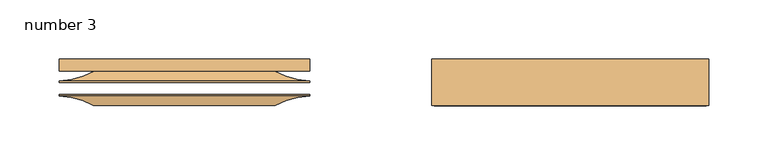
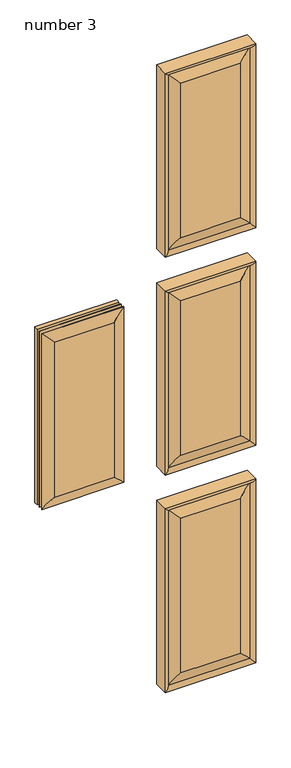
"""IFC4 building model written with IfcOpenShell, lengths in millimetres: door geometry, Door-Interior-Karona-K5660-6_Panel : number 3."""

from ifc_helpers import new_model, si_unit, frame, origin, place, context, project, spatial, polyline, ellipse_curve, source, transform, mapped, element, save
from ifc_brep_helpers import plane_surface, cylinder_surface, revolved_surface, advanced_brep


def number_3_2ed70dbe(model_context):
    return source(origin(), model_context, "Body", "AdvancedBrep", [
        advanced_brep(
        [(268.2748, 54.4576, 1893.8748), (268.2748, 54.4576, 1414.4752), (57.1627, 54.4576, 1414.4752), (57.1627, 54.4576, 1893.8748), (268.2748, 34.7218, 1893.8748), (268.2748, 36.0454899, 1893.8748), (57.1627, 36.0454899, 1893.8748), (57.1627, 34.7218, 1893.8748), (57.1627, 44.5515929, 1893.8748), (268.2748, 44.5515929, 1893.8748), (57.1627, 34.7218, 1414.4752), (57.1627, 36.0454899, 1414.4752), (268.2748, 36.0454899, 1414.4752), (268.2748, 34.7218, 1414.4752), (268.2748, 44.5515929, 1414.4752), (57.1627, 44.5515929, 1414.4752), (87.1686653, 44.5515929, 1863.8688347), (238.2688347, 44.5515929, 1863.8688347), (87.1686653, 44.5515929, 1444.4811653), (238.2688347, 44.5515929, 1444.4811653)],
        [
            (0, 1),
            (1, 2),
            (2, 3),
            (3, 0),
            (4, 5),
            (5, 6),
            (6, 7),
            (7, 4),
            (3, 8),
            (8, 9),
            (9, 0),
            (10, 11),
            (11, 12),
            (12, 13),
            (13, 10),
            (1, 14),
            (14, 15),
            (15, 2),
            (9, 14),
            (12, 5),
            (4, 13),
            (6, 11),
            (10, 7),
            (15, 8),
            (16, 6, ellipse_curve(frame((55.2243315, 100.0605261, 1895.8131685), z_axis=(-0.7071067811865475, 0.0, -0.7071067811865475), x_axis=(0.7071067811865476, 0.0, -0.7071067811865474)), 90.5724254, 64.0443762)),
            (5, 17, ellipse_curve(frame((270.2131685, 100.0605261, 1895.8131685), z_axis=(0.7071067811865475, 0.0, -0.7071067811865475), x_axis=(0.7071067811865476, 0.0, 0.7071067811865474)), 90.5724254, 64.0443762)),
            (17, 16),
            (18, 11, ellipse_curve(frame((55.2243315, 100.0605261, 1412.5368315), z_axis=(0.7071067811865475, 0.0, -0.7071067811865475), x_axis=(0.7071067811865474, 0.0, 0.7071067811865476)), 90.5724254, 64.0443762)),
            (16, 18),
            (19, 12, ellipse_curve(frame((270.2131685, 100.0605261, 1412.5368315), z_axis=(0.7071067811865475, 0.0, 0.7071067811865475), x_axis=(-0.7071067811865476, 0.0, 0.7071067811865474)), 90.5724254, 64.0443762)),
            (18, 19),
            (19, 17),
        ],
        [
            plane_surface(frame((57.1627, 54.4576, 1893.8748), z_axis=(0.0, 1.0, 0.0), x_axis=(0.0, 0.0, -1.0))),
            plane_surface(frame((57.1627, 34.7218, 1893.8748), z_axis=(0.0, 0.0, 1.0), x_axis=(-1.0, 0.0, 0.0))),
            plane_surface(frame((57.1627, 34.7218, 1414.4752), z_axis=(0.0, 0.0, -1.0), x_axis=(1.0, 0.0, 0.0))),
            plane_surface(frame((268.2748, 54.4576, 1893.8748), z_axis=(1.0, 0.0, 0.0), x_axis=(0.0, 0.0, -1.0))),
            plane_surface(frame((57.1627, 34.7218, 1893.8748), z_axis=(-1.0, 0.0, 0.0), x_axis=(0.0, 0.0, -1.0))),
            plane_surface(frame((268.2748, 34.7218, 1893.8748), z_axis=(0.0, -1.0, 0.0), x_axis=(0.0, 0.0, -1.0))),
            revolved_surface(polyline([(334.2575446888527, 100.0605261, 1831.7687923), (-8.820044688852704, 100.0605261, 1831.7687923)]), (279.4, 100.0605261, 1895.8131685), (1.0, 0.0, 0.0)),
            revolved_surface(polyline([(119.2687077, 100.0605261, 1959.8575446888528), (119.2687077, 100.0605261, 1348.4924553111473)]), (55.2243315, 100.0605261, 1905.0), (0.0, 0.0, 1.0)),
            revolved_surface(polyline([(-8.820044688852683, 100.0605261, 1476.5812077), (334.2575446888527, 100.0605261, 1476.5812077)]), (46.0375, 100.0605261, 1412.5368315), (-1.0, 0.0, 0.0)),
            revolved_surface(polyline([(206.1687923, 100.0605261, 1348.4924553111473), (206.1687923, 100.0605261, 1959.8575446888526)]), (270.2131685, 100.0605261, 1403.35), (0.0, 0.0, -1.0)),
            plane_surface(frame((279.4, 44.5515929, 1403.35), z_axis=(0.0, -1.0, 0.0), x_axis=(0.0, 0.0, 1.0))),
        ],
        [
            (0, [[1, 2, 3, 4]]),
            (1, [[5, 6, 7, 8]]),
            (1, [[9, 10, 11, -4]]),
            (2, [[12, 13, 14, 15]]),
            (2, [[16, 17, 18, -2]]),
            (3, [[-11, 19, -16, -1]]),
            (3, [[-14, 20, -5, 21]]),
            (4, [[-7, 22, -12, 23]]),
            (4, [[-18, 24, -9, -3]]),
            (5, [[-23, -15, -21, -8]]),
            (6, [[25, -6, 26, 27]]),
            (7, [[28, -22, -25, 29]]),
            (8, [[30, -13, -28, 31]]),
            (9, [[-26, -20, -30, 32]]),
            (10, [[-24, -17, -19, -10], [-32, -31, -29, -27]]),
        ],
    ),
        advanced_brep(
        [(268.2748, 24.6126, 1893.8748), (268.2748, 24.6126, 1414.4752), (57.1627, 24.6126, 1414.4752), (57.1627, 24.6126, 1893.8748), (239.4448579, 15.4432, 1443.3051421), (239.4448579, 15.4432, 1865.0448579), (85.9926421, 15.4432, 1865.0448579), (85.9926421, 15.4432, 1443.3051421), (57.1627, 23.2889101, 1893.8748), (268.2748, 23.2889101, 1893.8748), (268.2748, 23.2889101, 1414.4752), (57.1627, 23.2889101, 1414.4752)],
        [
            (0, 1),
            (1, 2),
            (2, 3),
            (3, 0),
            (4, 5),
            (5, 6),
            (6, 7),
            (7, 4),
            (3, 8),
            (8, 9),
            (9, 0),
            (1, 10),
            (10, 11),
            (11, 2),
            (7, 11, ellipse_curve(frame((55.2243315, -40.7261261, 1412.5368315), z_axis=(-0.7071067811865475, 0.0, 0.7071067811865475), x_axis=(-0.7071067811865476, 0.0, -0.7071067811865474)), 90.5724254, 64.0443762)),
            (10, 4, ellipse_curve(frame((270.2131685, -40.7261261, 1412.5368315), z_axis=(0.7071067811865475, 0.0, 0.7071067811865475), x_axis=(-0.7071067811865476, 0.0, 0.7071067811865474)), 90.5724254, 64.0443762)),
            (10, 9),
            (9, 5, ellipse_curve(frame((270.2131685, -40.7261261, 1895.8131685), z_axis=(-0.7071067811865475, 0.0, 0.7071067811865475), x_axis=(-0.7071067811865474, 0.0, -0.7071067811865476)), 90.5724254, 64.0443762)),
            (8, 6, ellipse_curve(frame((55.2243315, -40.7261261, 1895.8131685), z_axis=(-0.7071067811865475, 0.0, -0.7071067811865475), x_axis=(0.7071067811865476, 0.0, -0.7071067811865474)), 90.5724254, 64.0443762)),
            (8, 11),
        ],
        [
            plane_surface(frame((57.1627, 24.6126, 1893.8748), z_axis=(0.0, 1.0, 0.0), x_axis=(0.0, 0.0, -1.0))),
            plane_surface(frame((268.2748, 15.4432, 1893.8748), z_axis=(0.0, -1.0, 0.0), x_axis=(0.0, 0.0, -1.0))),
            plane_surface(frame((57.1627, 34.7218, 1893.8748), z_axis=(0.0, 0.0, 1.0), x_axis=(-1.0, 0.0, 0.0))),
            plane_surface(frame((57.1627, 34.7218, 1414.4752), z_axis=(0.0, 0.0, -1.0), x_axis=(1.0, 0.0, 0.0))),
            revolved_surface(polyline([(-8.820044688852711, -40.7261261, 1476.5812077), (334.2575446888527, -40.7261261, 1476.5812077)]), (46.0375, -40.7261261, 1412.5368315), (-1.0, 0.0, 0.0)),
            revolved_surface(polyline([(206.1687923, -40.7261261, 1348.4924553111473), (206.1687923, -40.7261261, 1959.8575446888528)]), (270.2131685, -40.7261261, 1403.35), (0.0, 0.0, -1.0)),
            revolved_surface(polyline([(334.2575446888527, -40.7261261, 1831.7687923), (-8.820044688852704, -40.7261261, 1831.7687923)]), (279.4, -40.7261261, 1895.8131685), (1.0, 0.0, 0.0)),
            revolved_surface(polyline([(119.2687077, -40.7261261, 1959.8575446888528), (119.2687077, -40.7261261, 1348.4924553111473)]), (55.2243315, -40.7261261, 1905.0), (0.0, 0.0, 1.0)),
            plane_surface(frame((268.2748, 24.6126, 1893.8748), z_axis=(1.0, 0.0, 0.0), x_axis=(0.0, 0.0, -1.0))),
            plane_surface(frame((57.1627, 15.4432, 1893.8748), z_axis=(-1.0, 0.0, 0.0), x_axis=(0.0, 0.0, -1.0))),
        ],
        [
            (0, [[1, 2, 3, 4]]),
            (1, [[5, 6, 7, 8]]),
            (2, [[9, 10, 11, -4]]),
            (3, [[12, 13, 14, -2]]),
            (4, [[-8, 15, -13, 16]]),
            (5, [[17, 18, -5, -16]]),
            (6, [[-10, 19, -6, -18]]),
            (7, [[20, -15, -7, -19]]),
            (8, [[-11, -17, -12, -1]]),
            (9, [[-14, -20, -9, -3]]),
        ],
    ),
        advanced_brep(
        [(279.4, 15.2908, 1905.0), (46.0375, 15.2908, 1905.0), (57.3628137, 24.6126, 1893.6746863), (268.0746863, 24.6126, 1893.6746863), (57.1627, 46.3324899, 1893.8748), (57.1627, 46.3324899, 1414.4752), (48.2727, 54.4576, 1405.5852), (48.2727, 54.4576, 1902.7648), (268.2748, 46.3324899, 1414.4752), (268.2748, 46.3324899, 1893.8748), (277.1648, 54.4576, 1902.7648), (277.1648, 54.4576, 1405.5852), (46.0375, 54.4576, 1403.35), (279.4, 54.4576, 1403.35), (279.4, 15.2908, 1403.35), (46.0375, 15.2908, 1403.35), (57.1627, 34.7218, 1414.4752), (268.2748, 34.7218, 1414.4752), (47.3075, 24.6126, 1903.73), (47.3075, 24.6126, 1404.62), (47.3075, 34.7218, 1404.62), (47.3075, 34.7218, 1903.73), (278.13, 24.6126, 1404.62), (278.13, 24.6126, 1903.73), (57.3628137, 24.6126, 1414.6753137), (268.0746863, 24.6126, 1414.6753137), (278.13, 34.7218, 1404.62), (279.4, 54.4576, 1905.0), (268.2748, 34.7218, 1893.8748), (278.13, 34.7218, 1903.73), (46.0375, 54.4576, 1905.0), (57.1627, 34.7218, 1893.8748)],
        [
            (0, 1),
            (1, 2, ellipse_curve(frame((47.0685124, 25.5788135, 1903.9689876), z_axis=(0.7071067811865475, 0.0, 0.7071067811865475), x_axis=(0.7071067811865476, 0.0, -0.7071067811865474)), 14.6223259, 10.3395458)),
            (2, 3),
            (3, 0, ellipse_curve(frame((278.3689876, 25.5788135, 1903.9689876), z_axis=(-0.7071067811865475, 0.0, 0.7071067811865475), x_axis=(0.7071067811865476, 0.0, 0.7071067811865474)), 14.6223259, 10.3395458)),
            (4, 5),
            (5, 6, ellipse_curve(frame((48.2727, 45.531597, 1405.5852), z_axis=(-0.7071067811865475, 0.0, 0.7071067811865475), x_axis=(0.7071067811865474, 0.0, 0.7071067811865476)), 12.6232745, 8.926003)),
            (6, 7),
            (7, 4, ellipse_curve(frame((48.2727, 45.531597, 1902.7648), z_axis=(-0.7071067811865475, 0.0, -0.7071067811865475), x_axis=(-0.7071067811865474, 0.0, 0.7071067811865476)), 12.6232745, 8.926003)),
            (8, 9),
            (9, 10, ellipse_curve(frame((277.1648, 45.531597, 1902.7648), z_axis=(0.7071067811865475, 0.0, -0.7071067811865475), x_axis=(-0.7071067811865474, 0.0, -0.7071067811865476)), 12.6232745, 8.926003)),
            (10, 11),
            (11, 8, ellipse_curve(frame((277.1648, 45.531597, 1405.5852), z_axis=(0.7071067811865475, 0.0, 0.7071067811865475), x_axis=(0.7071067811865474, 0.0, -0.7071067811865476)), 12.6232745, 8.926003)),
            (12, 13),
            (13, 14),
            (14, 15),
            (15, 12),
            (16, 17),
            (17, 8),
            (8, 5),
            (5, 16),
            (18, 19),
            (19, 20),
            (20, 21),
            (21, 18),
            (22, 19),
            (18, 23),
            (23, 22),
            (24, 25),
            (25, 3),
            (2, 24),
            (22, 26),
            (26, 20),
            (13, 27),
            (27, 0),
            (0, 14),
            (17, 28),
            (28, 9),
            (23, 29),
            (29, 26),
            (27, 30),
            (30, 1),
            (28, 31),
            (31, 4),
            (4, 9),
            (21, 29),
            (30, 12),
            (15, 1),
            (31, 16),
            (6, 11),
            (10, 7),
            (14, 25, ellipse_curve(frame((278.3689876, 25.5788135, 1404.3810124), z_axis=(-0.7071067811865475, 0.0, -0.7071067811865475), x_axis=(-0.7071067811865476, 0.0, 0.7071067811865474)), 14.6223259, 10.3395458)),
            (24, 15, ellipse_curve(frame((47.0685124, 25.5788135, 1404.3810124), z_axis=(0.7071067811865475, 0.0, -0.7071067811865475), x_axis=(-0.7071067811865476, 0.0, -0.7071067811865474)), 14.6223259, 10.3395458)),
        ],
        [
            cylinder_surface(frame((279.4, 25.5788135, 1903.9689876), z_axis=(1.0, 0.0, 0.0), x_axis=(0.0, -1.0, 0.0)), 10.3395458),
            cylinder_surface(frame((48.2727, 45.531597, 1905.0), z_axis=(0.0, 0.0, 1.0), x_axis=(0.0, -1.0, 0.0)), 8.926003),
            cylinder_surface(frame((277.1648, 45.531597, 1403.35), z_axis=(0.0, 0.0, -1.0), x_axis=(0.0, -1.0, 0.0)), 8.926003),
            plane_surface(frame((46.0375, 15.2908, 1403.35), z_axis=(0.0, 0.0, -1.0), x_axis=(1.0, 0.0, 0.0))),
            plane_surface(frame((57.1627, 46.3324899, 1414.4752), z_axis=(0.0, 0.0, 1.0), x_axis=(1.0, 0.0, 0.0))),
            plane_surface(frame((47.3075, 34.7218, 1903.73), z_axis=(1.0, 0.0, 0.0), x_axis=(0.0, 0.0, -1.0))),
            plane_surface(frame((47.3075, 24.6126, 1903.73), z_axis=(0.0, 1.0, 0.0), x_axis=(0.0, 0.0, -1.0))),
            plane_surface(frame((47.3075, 34.7218, 1404.62), z_axis=(0.0, 0.0, 1.0), x_axis=(1.0, 0.0, 0.0))),
            plane_surface(frame((279.4, 15.2908, 1403.35), z_axis=(1.0, 0.0, 0.0), x_axis=(0.0, 0.0, 1.0))),
            plane_surface(frame((268.2748, 46.3324899, 1414.4752), z_axis=(-1.0, 0.0, 0.0), x_axis=(0.0, 0.0, 1.0))),
            plane_surface(frame((278.13, 34.7218, 1404.62), z_axis=(-1.0, 0.0, 0.0), x_axis=(0.0, 0.0, 1.0))),
            plane_surface(frame((279.4, 15.2908, 1905.0), z_axis=(0.0, 0.0, 1.0), x_axis=(-1.0, 0.0, 0.0))),
            plane_surface(frame((268.2748, 46.3324899, 1893.8748), z_axis=(0.0, 0.0, -1.0), x_axis=(-1.0, 0.0, 0.0))),
            plane_surface(frame((278.13, 34.7218, 1903.73), z_axis=(0.0, 0.0, -1.0), x_axis=(-1.0, 0.0, 0.0))),
            plane_surface(frame((46.0375, 15.2908, 1905.0), z_axis=(-1.0, 0.0, 0.0), x_axis=(0.0, 0.0, -1.0))),
            plane_surface(frame((57.1627, 46.3324899, 1893.8748), z_axis=(1.0, 0.0, 0.0), x_axis=(0.0, 0.0, -1.0))),
            plane_surface(frame((57.1627, 34.7218, 1893.8748), z_axis=(0.0, -1.0, 0.0), x_axis=(0.0, 0.0, -1.0))),
            plane_surface(frame((46.0375, 54.4576, 1905.0), z_axis=(0.0, 1.0, 0.0), x_axis=(0.0, 0.0, -1.0))),
            cylinder_surface(frame((46.0375, 45.531597, 1405.5852), z_axis=(-1.0, 0.0, 0.0), x_axis=(0.0, -1.0, 0.0)), 8.926003),
            cylinder_surface(frame((46.0375, 25.5788135, 1404.3810124), z_axis=(-1.0, 0.0, 0.0), x_axis=(0.0, -1.0, 0.0)), 10.3395458),
            cylinder_surface(frame((278.3689876, 25.5788135, 1403.35), z_axis=(0.0, 0.0, -1.0), x_axis=(0.0, -1.0, 0.0)), 10.3395458),
            cylinder_surface(frame((279.4, 45.531597, 1902.7648), z_axis=(1.0, 0.0, 0.0), x_axis=(0.0, -1.0, 0.0)), 8.926003),
            cylinder_surface(frame((47.0685124, 25.5788135, 1905.0), z_axis=(0.0, 0.0, 1.0), x_axis=(0.0, -1.0, 0.0)), 10.3395458),
        ],
        [
            (0, [[1, 2, 3, 4]]),
            (1, [[5, 6, 7, 8]]),
            (2, [[9, 10, 11, 12]]),
            (3, [[13, 14, 15, 16]]),
            (4, [[17, 18, 19, 20]]),
            (5, [[21, 22, 23, 24]]),
            (6, [[25, -21, 26, 27], [28, 29, -3, 30]]),
            (7, [[-25, 31, 32, -22]]),
            (8, [[33, 34, 35, -14]]),
            (9, [[36, 37, -9, -18]]),
            (10, [[-27, 38, 39, -31]]),
            (11, [[40, 41, -1, -34]]),
            (12, [[42, 43, 44, -37]]),
            (13, [[-26, -24, 45, -38]]),
            (14, [[46, -16, 47, -41]]),
            (15, [[48, -20, -5, -43]]),
            (16, [[-32, -39, -45, -23], [-17, -48, -42, -36]]),
            (17, [[-13, -46, -40, -33], [49, -11, 50, -7]]),
            (18, [[-19, -12, -49, -6]]),
            (19, [[-15, 51, -28, 52]]),
            (20, [[-35, -4, -29, -51]]),
            (21, [[-44, -8, -50, -10]]),
            (22, [[-47, -52, -30, -2]]),
        ],
    ),
        advanced_brep(
        [(268.2748, 54.4576, 1300.1498), (268.2748, 54.4576, 820.7502), (57.1627, 54.4576, 820.7502), (57.1627, 54.4576, 1300.1498), (268.2748, 34.7218, 1300.1498), (268.2748, 36.0454899, 1300.1498), (57.1627, 36.0454899, 1300.1498), (57.1627, 34.7218, 1300.1498), (57.1627, 44.5515929, 1300.1498), (268.2748, 44.5515929, 1300.1498), (57.1627, 34.7218, 820.7502), (57.1627, 36.0454899, 820.7502), (268.2748, 36.0454899, 820.7502), (268.2748, 34.7218, 820.7502), (268.2748, 44.5515929, 820.7502), (57.1627, 44.5515929, 820.7502), (87.1686653, 44.5515929, 1270.1438347), (238.2688347, 44.5515929, 1270.1438347), (87.1686653, 44.5515929, 850.7561653), (238.2688347, 44.5515929, 850.7561653)],
        [
            (0, 1),
            (1, 2),
            (2, 3),
            (3, 0),
            (4, 5),
            (5, 6),
            (6, 7),
            (7, 4),
            (3, 8),
            (8, 9),
            (9, 0),
            (10, 11),
            (11, 12),
            (12, 13),
            (13, 10),
            (1, 14),
            (14, 15),
            (15, 2),
            (9, 14),
            (12, 5),
            (4, 13),
            (6, 11),
            (10, 7),
            (15, 8),
            (16, 6, ellipse_curve(frame((55.2243315, 100.0605261, 1302.0881685), z_axis=(-0.7071067811865475, 0.0, -0.7071067811865475), x_axis=(0.7071067811865476, 0.0, -0.7071067811865474)), 90.5724254, 64.0443762)),
            (5, 17, ellipse_curve(frame((270.2131685, 100.0605261, 1302.0881685), z_axis=(0.7071067811865475, 0.0, -0.7071067811865475), x_axis=(0.7071067811865476, 0.0, 0.7071067811865474)), 90.5724254, 64.0443762)),
            (17, 16),
            (18, 11, ellipse_curve(frame((55.2243315, 100.0605261, 818.8118315), z_axis=(0.7071067811865475, 0.0, -0.7071067811865475), x_axis=(0.7071067811865474, 0.0, 0.7071067811865476)), 90.5724254, 64.0443762)),
            (16, 18),
            (19, 12, ellipse_curve(frame((270.2131685, 100.0605261, 818.8118315), z_axis=(0.7071067811865475, 0.0, 0.7071067811865475), x_axis=(-0.7071067811865476, 0.0, 0.7071067811865474)), 90.5724254, 64.0443762)),
            (18, 19),
            (19, 17),
        ],
        [
            plane_surface(frame((57.1627, 54.4576, 1300.1498), z_axis=(0.0, 1.0, 0.0), x_axis=(0.0, 0.0, -1.0))),
            plane_surface(frame((57.1627, 34.7218, 1300.1498), z_axis=(0.0, 0.0, 1.0), x_axis=(-1.0, 0.0, 0.0))),
            plane_surface(frame((57.1627, 34.7218, 820.7502), z_axis=(0.0, 0.0, -1.0), x_axis=(1.0, 0.0, 0.0))),
            plane_surface(frame((268.2748, 54.4576, 1300.1498), z_axis=(1.0, 0.0, 0.0), x_axis=(0.0, 0.0, -1.0))),
            plane_surface(frame((57.1627, 34.7218, 1300.1498), z_axis=(-1.0, 0.0, 0.0), x_axis=(0.0, 0.0, -1.0))),
            plane_surface(frame((268.2748, 34.7218, 1300.1498), z_axis=(0.0, -1.0, 0.0), x_axis=(0.0, 0.0, -1.0))),
            revolved_surface(polyline([(334.2575446888527, 100.0605261, 1238.0437923), (-8.820044688852704, 100.0605261, 1238.0437923)]), (279.4, 100.0605261, 1302.0881685), (1.0, 0.0, 0.0)),
            revolved_surface(polyline([(119.2687077, 100.0605261, 1366.1325446888527), (119.2687077, 100.0605261, 754.7674553111474)]), (55.2243315, 100.0605261, 1311.275), (0.0, 0.0, 1.0)),
            revolved_surface(polyline([(-8.820044688852683, 100.0605261, 882.8562077), (334.2575446888527, 100.0605261, 882.8562077)]), (46.0375, 100.0605261, 818.8118315), (-1.0, 0.0, 0.0)),
            revolved_surface(polyline([(206.1687923, 100.0605261, 754.7674553111474), (206.1687923, 100.0605261, 1366.1325446888527)]), (270.2131685, 100.0605261, 809.625), (0.0, 0.0, -1.0)),
            plane_surface(frame((279.4, 44.5515929, 809.625), z_axis=(0.0, -1.0, 0.0), x_axis=(0.0, 0.0, 1.0))),
        ],
        [
            (0, [[1, 2, 3, 4]]),
            (1, [[5, 6, 7, 8]]),
            (1, [[9, 10, 11, -4]]),
            (2, [[12, 13, 14, 15]]),
            (2, [[16, 17, 18, -2]]),
            (3, [[-11, 19, -16, -1]]),
            (3, [[-14, 20, -5, 21]]),
            (4, [[-7, 22, -12, 23]]),
            (4, [[-18, 24, -9, -3]]),
            (5, [[-23, -15, -21, -8]]),
            (6, [[25, -6, 26, 27]]),
            (7, [[28, -22, -25, 29]]),
            (8, [[30, -13, -28, 31]]),
            (9, [[-26, -20, -30, 32]]),
            (10, [[-24, -17, -19, -10], [-32, -31, -29, -27]]),
        ],
    ),
        advanced_brep(
        [(268.2748, 24.6126, 1300.1498), (268.2748, 24.6126, 820.7502), (57.1627, 24.6126, 820.7502), (57.1627, 24.6126, 1300.1498), (239.4448579, 15.4432, 849.5801421), (239.4448579, 15.4432, 1271.3198579), (85.9926421, 15.4432, 1271.3198579), (85.9926421, 15.4432, 849.5801421), (57.1627, 23.2889101, 1300.1498), (268.2748, 23.2889101, 1300.1498), (268.2748, 23.2889101, 820.7502), (57.1627, 23.2889101, 820.7502)],
        [
            (0, 1),
            (1, 2),
            (2, 3),
            (3, 0),
            (4, 5),
            (5, 6),
            (6, 7),
            (7, 4),
            (3, 8),
            (8, 9),
            (9, 0),
            (1, 10),
            (10, 11),
            (11, 2),
            (7, 11, ellipse_curve(frame((55.2243315, -40.7261261, 818.8118315), z_axis=(-0.7071067811865475, 0.0, 0.7071067811865475), x_axis=(-0.7071067811865476, 0.0, -0.7071067811865474)), 90.5724254, 64.0443762)),
            (10, 4, ellipse_curve(frame((270.2131685, -40.7261261, 818.8118315), z_axis=(0.7071067811865475, 0.0, 0.7071067811865475), x_axis=(-0.7071067811865476, 0.0, 0.7071067811865474)), 90.5724254, 64.0443762)),
            (10, 9),
            (9, 5, ellipse_curve(frame((270.2131685, -40.7261261, 1302.0881685), z_axis=(-0.7071067811865475, 0.0, 0.7071067811865475), x_axis=(-0.7071067811865474, 0.0, -0.7071067811865476)), 90.5724254, 64.0443762)),
            (8, 6, ellipse_curve(frame((55.2243315, -40.7261261, 1302.0881685), z_axis=(-0.7071067811865475, 0.0, -0.7071067811865475), x_axis=(0.7071067811865476, 0.0, -0.7071067811865474)), 90.5724254, 64.0443762)),
            (8, 11),
        ],
        [
            plane_surface(frame((57.1627, 24.6126, 1300.1498), z_axis=(0.0, 1.0, 0.0), x_axis=(0.0, 0.0, -1.0))),
            plane_surface(frame((268.2748, 15.4432, 1300.1498), z_axis=(0.0, -1.0, 0.0), x_axis=(0.0, 0.0, -1.0))),
            plane_surface(frame((57.1627, 34.7218, 1300.1498), z_axis=(0.0, 0.0, 1.0), x_axis=(-1.0, 0.0, 0.0))),
            plane_surface(frame((57.1627, 34.7218, 820.7502), z_axis=(0.0, 0.0, -1.0), x_axis=(1.0, 0.0, 0.0))),
            revolved_surface(polyline([(-8.820044688852711, -40.7261261, 882.8562077), (334.2575446888527, -40.7261261, 882.8562077)]), (46.0375, -40.7261261, 818.8118315), (-1.0, 0.0, 0.0)),
            revolved_surface(polyline([(206.1687923, -40.7261261, 754.7674553111474), (206.1687923, -40.7261261, 1366.1325446888527)]), (270.2131685, -40.7261261, 809.625), (0.0, 0.0, -1.0)),
            revolved_surface(polyline([(334.2575446888527, -40.7261261, 1238.0437923), (-8.820044688852704, -40.7261261, 1238.0437923)]), (279.4, -40.7261261, 1302.0881685), (1.0, 0.0, 0.0)),
            revolved_surface(polyline([(119.2687077, -40.7261261, 1366.1325446888527), (119.2687077, -40.7261261, 754.7674553111474)]), (55.2243315, -40.7261261, 1311.275), (0.0, 0.0, 1.0)),
            plane_surface(frame((268.2748, 24.6126, 1300.1498), z_axis=(1.0, 0.0, 0.0), x_axis=(0.0, 0.0, -1.0))),
            plane_surface(frame((57.1627, 15.4432, 1300.1498), z_axis=(-1.0, 0.0, 0.0), x_axis=(0.0, 0.0, -1.0))),
        ],
        [
            (0, [[1, 2, 3, 4]]),
            (1, [[5, 6, 7, 8]]),
            (2, [[9, 10, 11, -4]]),
            (3, [[12, 13, 14, -2]]),
            (4, [[-8, 15, -13, 16]]),
            (5, [[17, 18, -5, -16]]),
            (6, [[-10, 19, -6, -18]]),
            (7, [[20, -15, -7, -19]]),
            (8, [[-11, -17, -12, -1]]),
            (9, [[-14, -20, -9, -3]]),
        ],
    ),
        advanced_brep(
        [(279.4, 15.2908, 1311.275), (46.0375, 15.2908, 1311.275), (57.3628137, 24.6126, 1299.9496863), (268.0746863, 24.6126, 1299.9496863), (57.1627, 46.3324899, 1300.1498), (57.1627, 46.3324899, 820.7502), (48.2727, 54.4576, 811.8602), (48.2727, 54.4576, 1309.0398), (268.2748, 46.3324899, 820.7502), (268.2748, 46.3324899, 1300.1498), (277.1648, 54.4576, 1309.0398), (277.1648, 54.4576, 811.8602), (46.0375, 54.4576, 809.625), (279.4, 54.4576, 809.625), (279.4, 15.2908, 809.625), (46.0375, 15.2908, 809.625), (57.1627, 34.7218, 820.7502), (268.2748, 34.7218, 820.7502), (47.3075, 24.6126, 1310.005), (47.3075, 24.6126, 810.895), (47.3075, 34.7218, 810.895), (47.3075, 34.7218, 1310.005), (278.13, 24.6126, 810.895), (278.13, 24.6126, 1310.005), (57.3628137, 24.6126, 820.9503137), (268.0746863, 24.6126, 820.9503137), (278.13, 34.7218, 810.895), (279.4, 54.4576, 1311.275), (268.2748, 34.7218, 1300.1498), (278.13, 34.7218, 1310.005), (46.0375, 54.4576, 1311.275), (57.1627, 34.7218, 1300.1498)],
        [
            (0, 1),
            (1, 2, ellipse_curve(frame((47.0685124, 25.5788135, 1310.2439876), z_axis=(0.7071067811865475, 0.0, 0.7071067811865475), x_axis=(0.7071067811865476, 0.0, -0.7071067811865474)), 14.6223259, 10.3395458)),
            (2, 3),
            (3, 0, ellipse_curve(frame((278.3689876, 25.5788135, 1310.2439876), z_axis=(-0.7071067811865475, 0.0, 0.7071067811865475), x_axis=(0.7071067811865476, 0.0, 0.7071067811865474)), 14.6223259, 10.3395458)),
            (4, 5),
            (5, 6, ellipse_curve(frame((48.2727, 45.531597, 811.8602), z_axis=(-0.7071067811865475, 0.0, 0.7071067811865475), x_axis=(0.7071067811865474, 0.0, 0.7071067811865476)), 12.6232745, 8.926003)),
            (6, 7),
            (7, 4, ellipse_curve(frame((48.2727, 45.531597, 1309.0398), z_axis=(-0.7071067811865475, 0.0, -0.7071067811865475), x_axis=(-0.7071067811865474, 0.0, 0.7071067811865476)), 12.6232745, 8.926003)),
            (8, 9),
            (9, 10, ellipse_curve(frame((277.1648, 45.531597, 1309.0398), z_axis=(0.7071067811865475, 0.0, -0.7071067811865475), x_axis=(-0.7071067811865474, 0.0, -0.7071067811865476)), 12.6232745, 8.926003)),
            (10, 11),
            (11, 8, ellipse_curve(frame((277.1648, 45.531597, 811.8602), z_axis=(0.7071067811865475, 0.0, 0.7071067811865475), x_axis=(0.7071067811865474, 0.0, -0.7071067811865476)), 12.6232745, 8.926003)),
            (12, 13),
            (13, 14),
            (14, 15),
            (15, 12),
            (16, 17),
            (17, 8),
            (8, 5),
            (5, 16),
            (18, 19),
            (19, 20),
            (20, 21),
            (21, 18),
            (22, 19),
            (18, 23),
            (23, 22),
            (24, 25),
            (25, 3),
            (2, 24),
            (14, 25, ellipse_curve(frame((278.3689876, 25.5788135, 810.6560124), z_axis=(-0.7071067811865475, 0.0, -0.7071067811865475), x_axis=(-0.7071067811865476, 0.0, 0.7071067811865474)), 14.6223259, 10.3395458)),
            (24, 15, ellipse_curve(frame((47.0685124, 25.5788135, 810.6560124), z_axis=(0.7071067811865475, 0.0, -0.7071067811865475), x_axis=(-0.7071067811865476, 0.0, -0.7071067811865474)), 14.6223259, 10.3395458)),
            (22, 26),
            (26, 20),
            (13, 27),
            (27, 0),
            (0, 14),
            (17, 28),
            (28, 9),
            (23, 29),
            (29, 26),
            (27, 30),
            (30, 1),
            (28, 31),
            (31, 4),
            (4, 9),
            (21, 29),
            (30, 12),
            (15, 1),
            (31, 16),
            (6, 11),
            (10, 7),
        ],
        [
            cylinder_surface(frame((279.4, 25.5788135, 1310.2439876), z_axis=(1.0, 0.0, 0.0), x_axis=(0.0, -1.0, 0.0)), 10.3395458),
            cylinder_surface(frame((48.2727, 45.531597, 1311.275), z_axis=(0.0, 0.0, 1.0), x_axis=(0.0, -1.0, 0.0)), 8.926003),
            cylinder_surface(frame((277.1648, 45.531597, 809.625), z_axis=(0.0, 0.0, -1.0), x_axis=(0.0, -1.0, 0.0)), 8.926003),
            plane_surface(frame((46.0375, 15.2908, 809.625), z_axis=(0.0, 0.0, -1.0), x_axis=(1.0, 0.0, 0.0))),
            plane_surface(frame((57.1627, 46.3324899, 820.7502), z_axis=(0.0, 0.0, 1.0), x_axis=(1.0, 0.0, 0.0))),
            plane_surface(frame((47.3075, 34.7218, 1310.005), z_axis=(1.0, 0.0, 0.0), x_axis=(0.0, 0.0, -1.0))),
            plane_surface(frame((47.3075, 24.6126, 1310.005), z_axis=(0.0, 1.0, 0.0), x_axis=(0.0, 0.0, -1.0))),
            cylinder_surface(frame((46.0375, 25.5788135, 810.6560124), z_axis=(-1.0, 0.0, 0.0), x_axis=(0.0, -1.0, 0.0)), 10.3395458),
            plane_surface(frame((47.3075, 34.7218, 810.895), z_axis=(0.0, 0.0, 1.0), x_axis=(1.0, 0.0, 0.0))),
            plane_surface(frame((279.4, 15.2908, 809.625), z_axis=(1.0, 0.0, 0.0), x_axis=(0.0, 0.0, 1.0))),
            plane_surface(frame((268.2748, 46.3324899, 820.7502), z_axis=(-1.0, 0.0, 0.0), x_axis=(0.0, 0.0, 1.0))),
            plane_surface(frame((278.13, 34.7218, 810.895), z_axis=(-1.0, 0.0, 0.0), x_axis=(0.0, 0.0, 1.0))),
            plane_surface(frame((279.4, 15.2908, 1311.275), z_axis=(0.0, 0.0, 1.0), x_axis=(-1.0, 0.0, 0.0))),
            plane_surface(frame((268.2748, 46.3324899, 1300.1498), z_axis=(0.0, 0.0, -1.0), x_axis=(-1.0, 0.0, 0.0))),
            plane_surface(frame((278.13, 34.7218, 1310.005), z_axis=(0.0, 0.0, -1.0), x_axis=(-1.0, 0.0, 0.0))),
            plane_surface(frame((46.0375, 15.2908, 1311.275), z_axis=(-1.0, 0.0, 0.0), x_axis=(0.0, 0.0, -1.0))),
            plane_surface(frame((57.1627, 46.3324899, 1300.1498), z_axis=(1.0, 0.0, 0.0), x_axis=(0.0, 0.0, -1.0))),
            plane_surface(frame((57.1627, 34.7218, 1300.1498), z_axis=(0.0, -1.0, 0.0), x_axis=(0.0, 0.0, -1.0))),
            plane_surface(frame((46.0375, 54.4576, 1311.275), z_axis=(0.0, 1.0, 0.0), x_axis=(0.0, 0.0, -1.0))),
            cylinder_surface(frame((46.0375, 45.531597, 811.8602), z_axis=(-1.0, 0.0, 0.0), x_axis=(0.0, -1.0, 0.0)), 8.926003),
            cylinder_surface(frame((278.3689876, 25.5788135, 809.625), z_axis=(0.0, 0.0, -1.0), x_axis=(0.0, -1.0, 0.0)), 10.3395458),
            cylinder_surface(frame((279.4, 45.531597, 1309.0398), z_axis=(1.0, 0.0, 0.0), x_axis=(0.0, -1.0, 0.0)), 8.926003),
            cylinder_surface(frame((47.0685124, 25.5788135, 1311.275), z_axis=(0.0, 0.0, 1.0), x_axis=(0.0, -1.0, 0.0)), 10.3395458),
        ],
        [
            (0, [[1, 2, 3, 4]]),
            (1, [[5, 6, 7, 8]]),
            (2, [[9, 10, 11, 12]]),
            (3, [[13, 14, 15, 16]]),
            (4, [[17, 18, 19, 20]]),
            (5, [[21, 22, 23, 24]]),
            (6, [[25, -21, 26, 27], [28, 29, -3, 30]]),
            (7, [[-15, 31, -28, 32]]),
            (8, [[-25, 33, 34, -22]]),
            (9, [[35, 36, 37, -14]]),
            (10, [[38, 39, -9, -18]]),
            (11, [[-27, 40, 41, -33]]),
            (12, [[42, 43, -1, -36]]),
            (13, [[44, 45, 46, -39]]),
            (14, [[-26, -24, 47, -40]]),
            (15, [[48, -16, 49, -43]]),
            (16, [[50, -20, -5, -45]]),
            (17, [[-34, -41, -47, -23], [-17, -50, -44, -38]]),
            (18, [[-13, -48, -42, -35], [51, -11, 52, -7]]),
            (19, [[-19, -12, -51, -6]]),
            (20, [[-37, -4, -29, -31]]),
            (21, [[-46, -8, -52, -10]]),
            (22, [[-49, -32, -30, -2]]),
        ],
    ),
        advanced_brep(
        [(268.2748, 54.4576, 706.4248), (268.2748, 54.4576, 227.0252), (57.1627, 54.4576, 227.0252), (57.1627, 54.4576, 706.4248), (268.2748, 34.7218, 706.4248), (268.2748, 36.0454899, 706.4248), (57.1627, 36.0454899, 706.4248), (57.1627, 34.7218, 706.4248), (57.1627, 44.5515929, 706.4248), (268.2748, 44.5515929, 706.4248), (57.1627, 34.7218, 227.0252), (57.1627, 36.0454899, 227.0252), (268.2748, 36.0454899, 227.0252), (268.2748, 34.7218, 227.0252), (268.2748, 44.5515929, 227.0252), (57.1627, 44.5515929, 227.0252), (87.1686653, 44.5515929, 676.4188347), (238.2688347, 44.5515929, 676.4188347), (87.1686653, 44.5515929, 257.0311653), (238.2688347, 44.5515929, 257.0311653)],
        [
            (0, 1),
            (1, 2),
            (2, 3),
            (3, 0),
            (4, 5),
            (5, 6),
            (6, 7),
            (7, 4),
            (3, 8),
            (8, 9),
            (9, 0),
            (10, 11),
            (11, 12),
            (12, 13),
            (13, 10),
            (1, 14),
            (14, 15),
            (15, 2),
            (9, 14),
            (12, 5),
            (4, 13),
            (6, 11),
            (10, 7),
            (15, 8),
            (16, 6, ellipse_curve(frame((55.2243315, 100.0605261, 708.3631685), z_axis=(-0.7071067811865475, 0.0, -0.7071067811865475), x_axis=(0.7071067811865476, 0.0, -0.7071067811865474)), 90.5724254, 64.0443762)),
            (5, 17, ellipse_curve(frame((270.2131685, 100.0605261, 708.3631685), z_axis=(0.7071067811865475, 0.0, -0.7071067811865475), x_axis=(0.7071067811865476, 0.0, 0.7071067811865474)), 90.5724254, 64.0443762)),
            (17, 16),
            (18, 11, ellipse_curve(frame((55.2243315, 100.0605261, 225.0868315), z_axis=(0.7071067811865475, 0.0, -0.7071067811865475), x_axis=(0.7071067811865474, 0.0, 0.7071067811865476)), 90.5724254, 64.0443762)),
            (16, 18),
            (19, 12, ellipse_curve(frame((270.2131685, 100.0605261, 225.0868315), z_axis=(0.7071067811865475, 0.0, 0.7071067811865475), x_axis=(-0.7071067811865476, 0.0, 0.7071067811865474)), 90.5724254, 64.0443762)),
            (18, 19),
            (19, 17),
        ],
        [
            plane_surface(frame((57.1627, 54.4576, 706.4248), z_axis=(0.0, 1.0, 0.0), x_axis=(0.0, 0.0, -1.0))),
            plane_surface(frame((57.1627, 34.7218, 706.4248), z_axis=(0.0, 0.0, 1.0), x_axis=(-1.0, 0.0, 0.0))),
            plane_surface(frame((57.1627, 34.7218, 227.0252), z_axis=(0.0, 0.0, -1.0), x_axis=(1.0, 0.0, 0.0))),
            plane_surface(frame((268.2748, 54.4576, 706.4248), z_axis=(1.0, 0.0, 0.0), x_axis=(0.0, 0.0, -1.0))),
            plane_surface(frame((57.1627, 34.7218, 706.4248), z_axis=(-1.0, 0.0, 0.0), x_axis=(0.0, 0.0, -1.0))),
            plane_surface(frame((268.2748, 34.7218, 706.4248), z_axis=(0.0, -1.0, 0.0), x_axis=(0.0, 0.0, -1.0))),
            revolved_surface(polyline([(334.2575446888527, 100.0605261, 644.3187923), (-8.820044688852704, 100.0605261, 644.3187923)]), (279.4, 100.0605261, 708.3631685), (1.0, 0.0, 0.0)),
            revolved_surface(polyline([(119.2687077, 100.0605261, 772.4075446888527), (119.2687077, 100.0605261, 161.04245531114725)]), (55.2243315, 100.0605261, 717.55), (0.0, 0.0, 1.0)),
            revolved_surface(polyline([(-8.820044688852683, 100.0605261, 289.1312077), (334.2575446888527, 100.0605261, 289.1312077)]), (46.0375, 100.0605261, 225.0868315), (-1.0, 0.0, 0.0)),
            revolved_surface(polyline([(206.1687923, 100.0605261, 161.0424553111473), (206.1687923, 100.0605261, 772.4075446888527)]), (270.2131685, 100.0605261, 215.9), (0.0, 0.0, -1.0)),
            plane_surface(frame((279.4, 44.5515929, 215.9), z_axis=(0.0, -1.0, 0.0), x_axis=(0.0, 0.0, 1.0))),
        ],
        [
            (0, [[1, 2, 3, 4]]),
            (1, [[5, 6, 7, 8]]),
            (1, [[9, 10, 11, -4]]),
            (2, [[12, 13, 14, 15]]),
            (2, [[16, 17, 18, -2]]),
            (3, [[-11, 19, -16, -1]]),
            (3, [[-14, 20, -5, 21]]),
            (4, [[-7, 22, -12, 23]]),
            (4, [[-18, 24, -9, -3]]),
            (5, [[-23, -15, -21, -8]]),
            (6, [[25, -6, 26, 27]]),
            (7, [[28, -22, -25, 29]]),
            (8, [[30, -13, -28, 31]]),
            (9, [[-26, -20, -30, 32]]),
            (10, [[-24, -17, -19, -10], [-32, -31, -29, -27]]),
        ],
    ),
        advanced_brep(
        [(268.2748, 24.6126, 706.4248), (268.2748, 24.6126, 227.0252), (57.1627, 24.6126, 227.0252), (57.1627, 24.6126, 706.4248), (239.4448579, 15.4432, 255.8551421), (239.4448579, 15.4432, 677.5948579), (85.9926421, 15.4432, 677.5948579), (85.9926421, 15.4432, 255.8551421), (57.1627, 23.2889101, 706.4248), (268.2748, 23.2889101, 706.4248), (268.2748, 23.2889101, 227.0252), (57.1627, 23.2889101, 227.0252)],
        [
            (0, 1),
            (1, 2),
            (2, 3),
            (3, 0),
            (4, 5),
            (5, 6),
            (6, 7),
            (7, 4),
            (3, 8),
            (8, 9),
            (9, 0),
            (1, 10),
            (10, 11),
            (11, 2),
            (7, 11, ellipse_curve(frame((55.2243315, -40.7261261, 225.0868315), z_axis=(-0.7071067811865475, 0.0, 0.7071067811865475), x_axis=(-0.7071067811865476, 0.0, -0.7071067811865474)), 90.5724254, 64.0443762)),
            (10, 4, ellipse_curve(frame((270.2131685, -40.7261261, 225.0868315), z_axis=(0.7071067811865475, 0.0, 0.7071067811865475), x_axis=(-0.7071067811865476, 0.0, 0.7071067811865474)), 90.5724254, 64.0443762)),
            (10, 9),
            (9, 5, ellipse_curve(frame((270.2131685, -40.7261261, 708.3631685), z_axis=(-0.7071067811865475, 0.0, 0.7071067811865475), x_axis=(-0.7071067811865474, 0.0, -0.7071067811865476)), 90.5724254, 64.0443762)),
            (8, 6, ellipse_curve(frame((55.2243315, -40.7261261, 708.3631685), z_axis=(-0.7071067811865475, 0.0, -0.7071067811865475), x_axis=(0.7071067811865476, 0.0, -0.7071067811865474)), 90.5724254, 64.0443762)),
            (8, 11),
        ],
        [
            plane_surface(frame((57.1627, 24.6126, 706.4248), z_axis=(0.0, 1.0, 0.0), x_axis=(0.0, 0.0, -1.0))),
            plane_surface(frame((268.2748, 15.4432, 706.4248), z_axis=(0.0, -1.0, 0.0), x_axis=(0.0, 0.0, -1.0))),
            plane_surface(frame((57.1627, 34.7218, 706.4248), z_axis=(0.0, 0.0, 1.0), x_axis=(-1.0, 0.0, 0.0))),
            plane_surface(frame((57.1627, 34.7218, 227.0252), z_axis=(0.0, 0.0, -1.0), x_axis=(1.0, 0.0, 0.0))),
            revolved_surface(polyline([(-8.820044688852711, -40.7261261, 289.1312077), (334.2575446888527, -40.7261261, 289.1312077)]), (46.0375, -40.7261261, 225.0868315), (-1.0, 0.0, 0.0)),
            revolved_surface(polyline([(206.1687923, -40.7261261, 161.0424553111473), (206.1687923, -40.7261261, 772.4075446888527)]), (270.2131685, -40.7261261, 215.9), (0.0, 0.0, -1.0)),
            revolved_surface(polyline([(334.2575446888527, -40.7261261, 644.3187923), (-8.820044688852704, -40.7261261, 644.3187923)]), (279.4, -40.7261261, 708.3631685), (1.0, 0.0, 0.0)),
            revolved_surface(polyline([(119.2687077, -40.7261261, 772.4075446888527), (119.2687077, -40.7261261, 161.04245531114736)]), (55.2243315, -40.7261261, 717.55), (0.0, 0.0, 1.0)),
            plane_surface(frame((268.2748, 24.6126, 706.4248), z_axis=(1.0, 0.0, 0.0), x_axis=(0.0, 0.0, -1.0))),
            plane_surface(frame((57.1627, 15.4432, 706.4248), z_axis=(-1.0, 0.0, 0.0), x_axis=(0.0, 0.0, -1.0))),
        ],
        [
            (0, [[1, 2, 3, 4]]),
            (1, [[5, 6, 7, 8]]),
            (2, [[9, 10, 11, -4]]),
            (3, [[12, 13, 14, -2]]),
            (4, [[-8, 15, -13, 16]]),
            (5, [[17, 18, -5, -16]]),
            (6, [[-10, 19, -6, -18]]),
            (7, [[20, -15, -7, -19]]),
            (8, [[-11, -17, -12, -1]]),
            (9, [[-14, -20, -9, -3]]),
        ],
    ),
        advanced_brep(
        [(279.4, 15.2908, 717.55), (46.0375, 15.2908, 717.55), (57.3628137, 24.6126, 706.2246863), (268.0746863, 24.6126, 706.2246863), (57.1627, 46.3324899, 706.4248), (57.1627, 46.3324899, 227.0252), (48.2727, 54.4576, 218.1352), (48.2727, 54.4576, 715.3148), (268.2748, 46.3324899, 227.0252), (268.2748, 46.3324899, 706.4248), (277.1648, 54.4576, 715.3148), (277.1648, 54.4576, 218.1352), (46.0375, 54.4576, 215.9), (279.4, 54.4576, 215.9), (279.4, 15.2908, 215.9), (46.0375, 15.2908, 215.9), (57.1627, 34.7218, 227.0252), (268.2748, 34.7218, 227.0252), (47.3075, 24.6126, 716.28), (47.3075, 24.6126, 217.17), (47.3075, 34.7218, 217.17), (47.3075, 34.7218, 716.28), (278.13, 24.6126, 217.17), (278.13, 24.6126, 716.28), (57.3628137, 24.6126, 227.2253137), (268.0746863, 24.6126, 227.2253137), (278.13, 34.7218, 217.17), (279.4, 54.4576, 717.55), (268.2748, 34.7218, 706.4248), (278.13, 34.7218, 716.28), (46.0375, 54.4576, 717.55), (57.1627, 34.7218, 706.4248)],
        [
            (0, 1),
            (1, 2, ellipse_curve(frame((47.0685124, 25.5788135, 716.5189876), z_axis=(0.7071067811865475, 0.0, 0.7071067811865475), x_axis=(0.7071067811865476, 0.0, -0.7071067811865474)), 14.6223259, 10.3395458)),
            (2, 3),
            (3, 0, ellipse_curve(frame((278.3689876, 25.5788135, 716.5189876), z_axis=(-0.7071067811865475, 0.0, 0.7071067811865475), x_axis=(0.7071067811865476, 0.0, 0.7071067811865474)), 14.6223259, 10.3395458)),
            (4, 5),
            (5, 6, ellipse_curve(frame((48.2727, 45.531597, 218.1352), z_axis=(-0.7071067811865475, 0.0, 0.7071067811865475), x_axis=(0.7071067811865474, 0.0, 0.7071067811865476)), 12.6232745, 8.926003)),
            (6, 7),
            (7, 4, ellipse_curve(frame((48.2727, 45.531597, 715.3148), z_axis=(-0.7071067811865475, 0.0, -0.7071067811865475), x_axis=(-0.7071067811865474, 0.0, 0.7071067811865476)), 12.6232745, 8.926003)),
            (8, 9),
            (9, 10, ellipse_curve(frame((277.1648, 45.531597, 715.3148), z_axis=(0.7071067811865475, 0.0, -0.7071067811865475), x_axis=(-0.7071067811865474, 0.0, -0.7071067811865476)), 12.6232745, 8.926003)),
            (10, 11),
            (11, 8, ellipse_curve(frame((277.1648, 45.531597, 218.1352), z_axis=(0.7071067811865475, 0.0, 0.7071067811865475), x_axis=(0.7071067811865474, 0.0, -0.7071067811865476)), 12.6232745, 8.926003)),
            (12, 13),
            (13, 14),
            (14, 15),
            (15, 12),
            (16, 17),
            (17, 8),
            (8, 5),
            (5, 16),
            (18, 19),
            (19, 20),
            (20, 21),
            (21, 18),
            (22, 19),
            (18, 23),
            (23, 22),
            (24, 25),
            (25, 3),
            (2, 24),
            (14, 25, ellipse_curve(frame((278.3689876, 25.5788135, 216.9310124), z_axis=(-0.7071067811865475, 0.0, -0.7071067811865475), x_axis=(-0.7071067811865476, 0.0, 0.7071067811865474)), 14.6223259, 10.3395458)),
            (24, 15, ellipse_curve(frame((47.0685124, 25.5788135, 216.9310124), z_axis=(0.7071067811865475, 0.0, -0.7071067811865475), x_axis=(-0.7071067811865476, 0.0, -0.7071067811865474)), 14.6223259, 10.3395458)),
            (22, 26),
            (26, 20),
            (13, 27),
            (27, 0),
            (0, 14),
            (17, 28),
            (28, 9),
            (23, 29),
            (29, 26),
            (27, 30),
            (30, 1),
            (28, 31),
            (31, 4),
            (4, 9),
            (21, 29),
            (30, 12),
            (15, 1),
            (31, 16),
            (6, 11),
            (10, 7),
        ],
        [
            cylinder_surface(frame((279.4, 25.5788135, 716.5189876), z_axis=(1.0, 0.0, 0.0), x_axis=(0.0, -1.0, 0.0)), 10.3395458),
            cylinder_surface(frame((48.2727, 45.531597, 717.55), z_axis=(0.0, 0.0, 1.0), x_axis=(0.0, -1.0, 0.0)), 8.926003),
            cylinder_surface(frame((277.1648, 45.531597, 215.9), z_axis=(0.0, 0.0, -1.0), x_axis=(0.0, -1.0, 0.0)), 8.926003),
            plane_surface(frame((46.0375, 15.2908, 215.9), z_axis=(0.0, 0.0, -1.0), x_axis=(1.0, 0.0, 0.0))),
            plane_surface(frame((57.1627, 46.3324899, 227.0252), z_axis=(0.0, 0.0, 1.0), x_axis=(1.0, 0.0, 0.0))),
            plane_surface(frame((47.3075, 34.7218, 716.28), z_axis=(1.0, 0.0, 0.0), x_axis=(0.0, 0.0, -1.0))),
            plane_surface(frame((47.3075, 24.6126, 716.28), z_axis=(0.0, 1.0, 0.0), x_axis=(0.0, 0.0, -1.0))),
            cylinder_surface(frame((46.0375, 25.5788135, 216.9310124), z_axis=(-1.0, 0.0, 0.0), x_axis=(0.0, -1.0, 0.0)), 10.3395458),
            plane_surface(frame((47.3075, 34.7218, 217.17), z_axis=(0.0, 0.0, 1.0), x_axis=(1.0, 0.0, 0.0))),
            plane_surface(frame((279.4, 15.2908, 215.9), z_axis=(1.0, 0.0, 0.0), x_axis=(0.0, 0.0, 1.0))),
            plane_surface(frame((268.2748, 46.3324899, 227.0252), z_axis=(-1.0, 0.0, 0.0), x_axis=(0.0, 0.0, 1.0))),
            plane_surface(frame((278.13, 34.7218, 217.17), z_axis=(-1.0, 0.0, 0.0), x_axis=(0.0, 0.0, 1.0))),
            plane_surface(frame((279.4, 15.2908, 717.55), z_axis=(0.0, 0.0, 1.0), x_axis=(-1.0, 0.0, 0.0))),
            plane_surface(frame((268.2748, 46.3324899, 706.4248), z_axis=(0.0, 0.0, -1.0), x_axis=(-1.0, 0.0, 0.0))),
            plane_surface(frame((278.13, 34.7218, 716.28), z_axis=(0.0, 0.0, -1.0), x_axis=(-1.0, 0.0, 0.0))),
            plane_surface(frame((46.0375, 15.2908, 717.55), z_axis=(-1.0, 0.0, 0.0), x_axis=(0.0, 0.0, -1.0))),
            plane_surface(frame((57.1627, 46.3324899, 706.4248), z_axis=(1.0, 0.0, 0.0), x_axis=(0.0, 0.0, -1.0))),
            plane_surface(frame((57.1627, 34.7218, 706.4248), z_axis=(0.0, -1.0, 0.0), x_axis=(0.0, 0.0, -1.0))),
            plane_surface(frame((46.0375, 54.4576, 717.55), z_axis=(0.0, 1.0, 0.0), x_axis=(0.0, 0.0, -1.0))),
            cylinder_surface(frame((46.0375, 45.531597, 218.1352), z_axis=(-1.0, 0.0, 0.0), x_axis=(0.0, -1.0, 0.0)), 8.926003),
            cylinder_surface(frame((278.3689876, 25.5788135, 215.9), z_axis=(0.0, 0.0, -1.0), x_axis=(0.0, -1.0, 0.0)), 10.3395458),
            cylinder_surface(frame((279.4, 45.531597, 715.3148), z_axis=(1.0, 0.0, 0.0), x_axis=(0.0, -1.0, 0.0)), 8.926003),
            cylinder_surface(frame((47.0685124, 25.5788135, 717.55), z_axis=(0.0, 0.0, 1.0), x_axis=(0.0, -1.0, 0.0)), 10.3395458),
        ],
        [
            (0, [[1, 2, 3, 4]]),
            (1, [[5, 6, 7, 8]]),
            (2, [[9, 10, 11, 12]]),
            (3, [[13, 14, 15, 16]]),
            (4, [[17, 18, 19, 20]]),
            (5, [[21, 22, 23, 24]]),
            (6, [[25, -21, 26, 27], [28, 29, -3, 30]]),
            (7, [[-15, 31, -28, 32]]),
            (8, [[-25, 33, 34, -22]]),
            (9, [[35, 36, 37, -14]]),
            (10, [[38, 39, -9, -18]]),
            (11, [[-27, 40, 41, -33]]),
            (12, [[42, 43, -1, -36]]),
            (13, [[44, 45, 46, -39]]),
            (14, [[-26, -24, 47, -40]]),
            (15, [[48, -16, 49, -43]]),
            (16, [[50, -20, -5, -45]]),
            (17, [[-34, -41, -47, -23], [-17, -50, -44, -38]]),
            (18, [[-13, -48, -42, -35], [51, -11, 52, -7]]),
            (19, [[-19, -12, -51, -6]]),
            (20, [[-37, -4, -29, -31]]),
            (21, [[-46, -8, -52, -10]]),
            (22, [[-49, -32, -30, -2]]),
        ],
    ),
        advanced_brep(
        [(-268.2748, 54.4576, 1300.1498), (-57.1627, 54.4576, 1300.1498), (-57.1627, 54.4576, 820.7502), (-268.2748, 54.4576, 820.7502), (-268.2748, 34.7218, 1300.1498), (-57.1627, 34.7218, 1300.1498), (-57.1627, 36.0454899, 1300.1498), (-268.2748, 36.0454899, 1300.1498), (-268.2748, 44.5515929, 1300.1498), (-57.1627, 44.5515929, 1300.1498), (-57.1627, 34.7218, 820.7502), (-268.2748, 34.7218, 820.7502), (-268.2748, 36.0454899, 820.7502), (-57.1627, 36.0454899, 820.7502), (-57.1627, 44.5515929, 820.7502), (-268.2748, 44.5515929, 820.7502), (-87.1686653, 44.5515929, 1270.1438347), (-238.2688347, 44.5515929, 1270.1438347), (-87.1686653, 44.5515929, 850.7561653), (-238.2688347, 44.5515929, 850.7561653)],
        [
            (0, 1),
            (1, 2),
            (2, 3),
            (3, 0),
            (4, 5),
            (5, 6),
            (6, 7),
            (7, 4),
            (0, 8),
            (8, 9),
            (9, 1),
            (10, 11),
            (11, 12),
            (12, 13),
            (13, 10),
            (2, 14),
            (14, 15),
            (15, 3),
            (15, 8),
            (11, 4),
            (7, 12),
            (9, 14),
            (5, 10),
            (13, 6),
            (16, 17),
            (17, 7, ellipse_curve(frame((-270.2131685, 100.0605261, 1302.0881685), z_axis=(-0.7071067811865475, 0.0, -0.7071067811865475), x_axis=(-0.7071067811865476, 0.0, 0.7071067811865474)), 90.5724254, 64.0443762)),
            (6, 16, ellipse_curve(frame((-55.2243315, 100.0605261, 1302.0881685), z_axis=(0.7071067811865475, 0.0, -0.7071067811865475), x_axis=(-0.7071067811865476, 0.0, -0.7071067811865474)), 90.5724254, 64.0443762)),
            (18, 16),
            (13, 18, ellipse_curve(frame((-55.2243315, 100.0605261, 818.8118315), z_axis=(-0.7071067811865475, 0.0, -0.7071067811865475), x_axis=(-0.7071067811865474, 0.0, 0.7071067811865476)), 90.5724254, 64.0443762)),
            (19, 18),
            (12, 19, ellipse_curve(frame((-270.2131685, 100.0605261, 818.8118315), z_axis=(-0.7071067811865475, 0.0, 0.7071067811865475), x_axis=(0.7071067811865476, 0.0, 0.7071067811865474)), 90.5724254, 64.0443762)),
            (17, 19),
        ],
        [
            plane_surface(frame((-57.1627, 54.4576, 1300.1498), z_axis=(0.0, 1.0, 0.0), x_axis=(0.0, 0.0, -1.0))),
            plane_surface(frame((-57.1627, 34.7218, 1300.1498), z_axis=(0.0, 0.0, 1.0), x_axis=(1.0, 0.0, 0.0))),
            plane_surface(frame((-57.1627, 34.7218, 820.7502), z_axis=(0.0, 0.0, -1.0), x_axis=(-1.0, 0.0, 0.0))),
            plane_surface(frame((-268.2748, 54.4576, 1300.1498), z_axis=(-1.0, 0.0, 0.0), x_axis=(0.0, 0.0, -1.0))),
            plane_surface(frame((-57.1627, 34.7218, 1300.1498), z_axis=(1.0, 0.0, 0.0), x_axis=(0.0, 0.0, -1.0))),
            plane_surface(frame((-268.2748, 34.7218, 1300.1498), z_axis=(0.0, -1.0, 0.0), x_axis=(0.0, 0.0, -1.0))),
            revolved_surface(polyline([(-334.2575446888527, 100.0605261, 1238.0437923), (8.820044688852704, 100.0605261, 1238.0437923)]), (-279.4, 100.0605261, 1302.0881685), (-1.0, 0.0, 0.0)),
            revolved_surface(polyline([(-119.2687077, 100.0605261, 1366.1325446888527), (-119.2687077, 100.0605261, 754.7674553111474)]), (-55.2243315, 100.0605261, 1311.275), (0.0, 0.0, 1.0)),
            revolved_surface(polyline([(8.820044688852683, 100.0605261, 882.8562077), (-334.2575446888527, 100.0605261, 882.8562077)]), (-46.0375, 100.0605261, 818.8118315), (1.0, 0.0, 0.0)),
            revolved_surface(polyline([(-206.1687923, 100.0605261, 754.7674553111474), (-206.1687923, 100.0605261, 1366.1325446888527)]), (-270.2131685, 100.0605261, 809.625), (0.0, 0.0, -1.0)),
            plane_surface(frame((-279.4, 44.5515929, 809.625), z_axis=(0.0, -1.0, 0.0), x_axis=(0.0, 0.0, 1.0))),
        ],
        [
            (0, [[1, 2, 3, 4]]),
            (1, [[5, 6, 7, 8]]),
            (1, [[-1, 9, 10, 11]]),
            (2, [[12, 13, 14, 15]]),
            (2, [[-3, 16, 17, 18]]),
            (3, [[-4, -18, 19, -9]]),
            (3, [[20, -8, 21, -13]]),
            (4, [[-2, -11, 22, -16]]),
            (4, [[23, -15, 24, -6]]),
            (5, [[-5, -20, -12, -23]]),
            (6, [[25, 26, -7, 27]]),
            (7, [[28, -27, -24, 29]]),
            (8, [[30, -29, -14, 31]]),
            (9, [[32, -31, -21, -26]]),
            (10, [[-10, -19, -17, -22], [-25, -28, -30, -32]]),
        ],
    ),
        advanced_brep(
        [(-268.2748, 24.6126, 1300.1498), (-57.1627, 24.6126, 1300.1498), (-57.1627, 24.6126, 820.7502), (-268.2748, 24.6126, 820.7502), (-239.4448579, 15.4432, 849.5801421), (-85.9926421, 15.4432, 849.5801421), (-85.9926421, 15.4432, 1271.3198579), (-239.4448579, 15.4432, 1271.3198579), (-268.2748, 23.2889101, 1300.1498), (-57.1627, 23.2889101, 1300.1498), (-57.1627, 23.2889101, 820.7502), (-268.2748, 23.2889101, 820.7502)],
        [
            (0, 1),
            (1, 2),
            (2, 3),
            (3, 0),
            (4, 5),
            (5, 6),
            (6, 7),
            (7, 4),
            (0, 8),
            (8, 9),
            (9, 1),
            (2, 10),
            (10, 11),
            (11, 3),
            (4, 11, ellipse_curve(frame((-270.2131685, -40.7261261, 818.8118315), z_axis=(-0.7071067811865475, 0.0, 0.7071067811865475), x_axis=(0.7071067811865476, 0.0, 0.7071067811865474)), 90.5724254, 64.0443762)),
            (10, 5, ellipse_curve(frame((-55.2243315, -40.7261261, 818.8118315), z_axis=(0.7071067811865475, 0.0, 0.7071067811865475), x_axis=(0.7071067811865476, 0.0, -0.7071067811865474)), 90.5724254, 64.0443762)),
            (7, 8, ellipse_curve(frame((-270.2131685, -40.7261261, 1302.0881685), z_axis=(0.7071067811865475, 0.0, 0.7071067811865475), x_axis=(0.7071067811865474, 0.0, -0.7071067811865476)), 90.5724254, 64.0443762)),
            (8, 11),
            (6, 9, ellipse_curve(frame((-55.2243315, -40.7261261, 1302.0881685), z_axis=(0.7071067811865475, 0.0, -0.7071067811865475), x_axis=(-0.7071067811865476, 0.0, -0.7071067811865474)), 90.5724254, 64.0443762)),
            (10, 9),
        ],
        [
            plane_surface(frame((-57.1627, 24.6126, 1300.1498), z_axis=(0.0, 1.0, 0.0), x_axis=(0.0, 0.0, -1.0))),
            plane_surface(frame((-268.2748, 15.4432, 1300.1498), z_axis=(0.0, -1.0, 0.0), x_axis=(0.0, 0.0, -1.0))),
            plane_surface(frame((-57.1627, 34.7218, 1300.1498), z_axis=(0.0, 0.0, 1.0), x_axis=(1.0, 0.0, 0.0))),
            plane_surface(frame((-57.1627, 34.7218, 820.7502), z_axis=(0.0, 0.0, -1.0), x_axis=(-1.0, 0.0, 0.0))),
            revolved_surface(polyline([(8.820044688852711, -40.7261261, 882.8562077), (-334.2575446888527, -40.7261261, 882.8562077)]), (-46.0375, -40.7261261, 818.8118315), (1.0, 0.0, 0.0)),
            revolved_surface(polyline([(-206.1687923, -40.7261261, 754.7674553111474), (-206.1687923, -40.7261261, 1366.1325446888527)]), (-270.2131685, -40.7261261, 809.625), (0.0, 0.0, -1.0)),
            revolved_surface(polyline([(-334.2575446888527, -40.7261261, 1238.0437923), (8.820044688852704, -40.7261261, 1238.0437923)]), (-279.4, -40.7261261, 1302.0881685), (-1.0, 0.0, 0.0)),
            revolved_surface(polyline([(-119.2687077, -40.7261261, 1366.1325446888527), (-119.2687077, -40.7261261, 754.7674553111474)]), (-55.2243315, -40.7261261, 1311.275), (0.0, 0.0, 1.0)),
            plane_surface(frame((-268.2748, 24.6126, 1300.1498), z_axis=(-1.0, 0.0, 0.0), x_axis=(0.0, 0.0, -1.0))),
            plane_surface(frame((-57.1627, 15.4432, 1300.1498), z_axis=(1.0, 0.0, 0.0), x_axis=(0.0, 0.0, -1.0))),
        ],
        [
            (0, [[1, 2, 3, 4]]),
            (1, [[5, 6, 7, 8]]),
            (2, [[-1, 9, 10, 11]]),
            (3, [[-3, 12, 13, 14]]),
            (4, [[15, -13, 16, -5]]),
            (5, [[-15, -8, 17, 18]]),
            (6, [[-17, -7, 19, -10]]),
            (7, [[-19, -6, -16, 20]]),
            (8, [[-4, -14, -18, -9]]),
            (9, [[-2, -11, -20, -12]]),
        ],
    ),
    ])


if __name__ == "__main__":
    model = new_model("IFC4")
    model_context = context("Model", 3, world=origin())
    ifc_project = project(units=[si_unit("LENGTHUNIT", "METRE", prefix="MILLI")], contexts=[model_context])
    site = spatial("IfcSite", under=ifc_project)
    building = spatial("IfcBuilding", under=site)
    placement = place(None, origin())
    number_3_shape = number_3_2ed70dbe(model_context)
    element("IfcDoor", 1, ObjectType="Door-Interior-Karona-K5660-6_Panel : number 3", at=placement, inside=building, context=model_context, shape_type="MappedRepresentation", body=[
        mapped(number_3_shape, transform((0.0, 0.0, 0.0), x_axis=(1.0, 0.0, 0.0), y_axis=(0.0, 1.0, 0.0), z_axis=(0.0, 0.0, 1.0))),
    ])
    save(model, "model.ifc")

# Revit data of these elements
# Type "Door-Interior-Karona-K5660-6_Panel : number 3"
#   Type Mark = "83"
#   Youtube clip = ""
#   Warranty URL = "http://www.karonadoor.com/pdf/literature/Warranty_.pdf"
#   Warranty = "Limited lifetime warranty on all interior doors."
#   Uniformat II Description = ""
#   Uniformat II Code = ""
#   Uniclass 2015 Name = "Doorsets"
#   Uniclass 2015 Code = "Pr_30_59_24"
#   Uniclass 2.0 Description = "Doorsets"
#   Uniclass 2.0 Code = "PR-59-23"
#   Uniclass 1.4 Description = "Doors"
#   Uniclass 1.4 Code = "JL20"
#   URL = "http://www.karonadoor.com/"
#   UNSPSC Code = "30171511"
#   Technical description = "http://www.karonadoor.com/pdf/Architectural.Guide.pdf"
#   Support Email = "mailto:bimsupport@jeldwen.com"
#   Region South America = "None"
#   Region Oceania = "None"
#   Region North America = "CA, US"
#   Region Middle East = "None"
#   Region Europe = "None"
#   Region Asia = "None"
#   Region Antarctica = "None"
#   Region Africa = "None"
#   QR code = "http://bimobject.com/karona/product/K5660"
#   Product url = "http://www.karonadoor.com/commercial_products.php?category_id=1&style_id=1&image_id=21"
#   Product group = "Panel Doors"
#   Product family = "Commercial Products"
#   Product data url = "https://bimobject.com/karona/product/K5660"
#   Product certification = ""
#   Product SKU = "K5660"
#   Product Guid = "0ef6a8f4-4242-4391-b579-45df545b9ddd"
#   Operation = "Swing"
#   OmniClass Description = "Wood Doors"
#   OmniClass Code = "23-17 11 15"
#   NBS Reference Description = "Doorsets"
#   NBS Reference Code = "59-23"
#   Model = "K5660"
#   Material secondary = ""
#   Material main = "Wood"
#   Masterformat 2014 Description = "Stile and Rail Wood Doors"
#   Masterformat 2014 Code = "08 14 33"
#   Manufacturer name = "Karona"
#   Manufacturer country = "United States"
#   Manufacturer = "Karona Door, Inc."
#   Keynote = "08 14 33"
#   Installation instructions = ""
#   IFC Classification = "Door"
#   Green Product Information = "Available in Certified Wood, No-added Urea, & Recycled"
#   Fire Rating Data = "http://www.karonadoor.com/pdf/literature/Fire_Door_Options.pdf"
#   Fire Rating = "Available in 20, 45, 60, & 90 minute ratings."
#   EAN code = ""
#   Design country = "United States"
#   Description = "Commercial 6-Panel Stile and Rail Wood Door"
#   Date of publishing = ""
#   COBIe Type Category = ""
#   Brand url = "http://www.karonadoor.com/"
#   BIMobject main category code = "doors"
#   BIMobject main category = "Doors"
#   BIMobject category code = "doors-swing"
#   BIMobject category = "Swing"
#   Analytic Construction = "Solid core wood"
#   Sticking Profile Note = "Select only one sticking profile."
#   Sizing Statement = "Custom sizes are available."
#   Panel Style Note = "Select only one panel style."
#   Glass Options Note = "19 styles of glass are available."
#   Fire Door Note = "Available in 20, 45, 60, & 90 minute ratings."
#   Trim Width = 0' - 3 21/32"
#   Trim Reveal = 0' - 0 1/4"
#   Trim Offset = 0' - 3"
#   Top Rail Height = 0' - 5"
#   Thermal Resistance (R) = 0.382863 (m²·K)/W
#   Stile Width = 0' - 5"
#   Sticking Offset = 0' - 0 7/16"
#   Raised Panel Offset = 0' - 1 5/8"
#   Panel Height = 1' - 7 3/4"
#   Mullion Width = 0' - 3 5/8"
#   Mid Rail Height = 4' - 7 1/4"
#   Lock Rail Width = 0' - 3 5/8"
#   Lock Rail Height = 2' - 7 7/8"
#   Jamb to Door Gap = 0' - 0 3/64"
#   Hinge Length = 0' - 2 1/4"
#   Heat Transfer Coefficient (U) = 2.6120 W/(m²·K)
#   Daylight Opening Width = 0' - 0"
#   Daylight Opening Height = 0' - 0"
